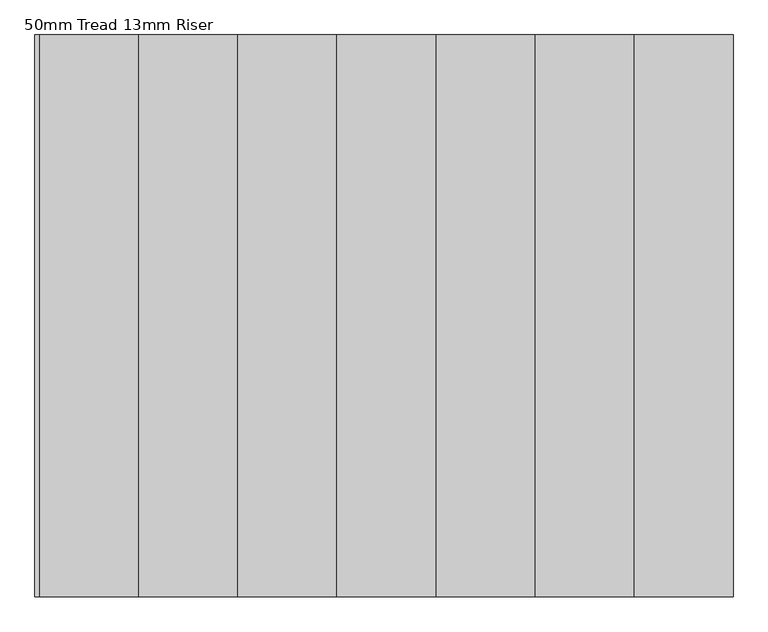
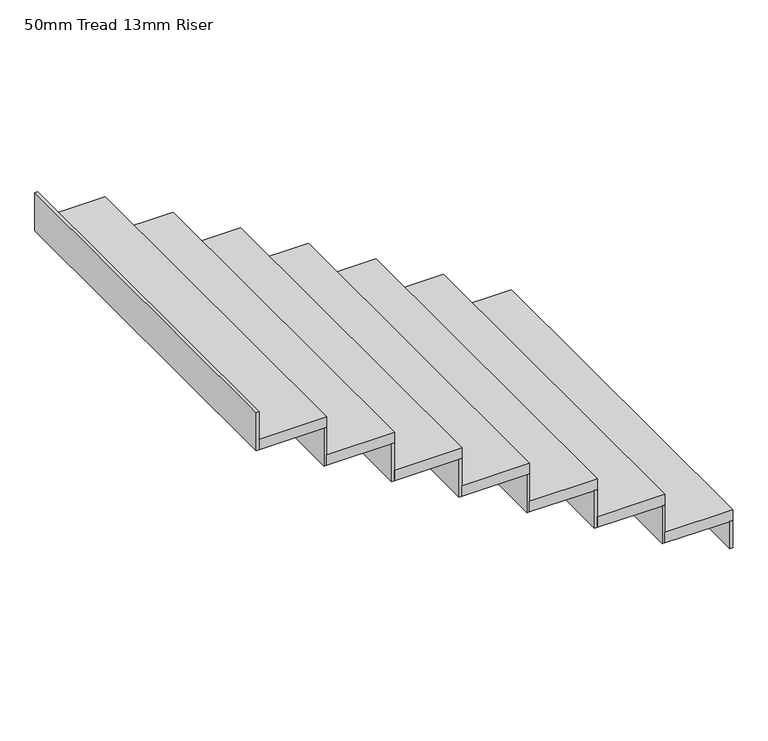
"""IFC4 building model written with IfcOpenShell, lengths in millimetres: stair flight geometry, 50mm Tread 13mm Riser."""

import ifcopenshell
import ifcopenshell.guid

model = None  # the IFC model being written
_history = None  # IfcOwnerHistory: only IFC2X3 demands one
_inside = {}  # id of a spatial element -> (the spatial element, [elements in it])
_under = {}  # id of a project, library or spatial element -> (it, [spatial elements below it])
_declared = {}  # id of a project -> (the project, [libraries it declares])
_typed = {}  # id of a type object -> (the type object, [elements of that type])
_made_of = {}  # id of a material, layer set ... -> (it, [elements and type objects made of it])


def new_model(schema):
    """Start an empty IFC model of exactly this schema.

    Asked for "IFC4X3", IfcOpenShell would pick the latest addendum, in which some entities
    have other attributes; the version numbers below select the first issue.
    IFC2X3 requires an IfcOwnerHistory on every rooted entity: one is made here for all.
    """
    global model, _history
    if schema == "IFC4X3":
        model = ifcopenshell.file(schema_version=(4, 3, 0, 0))
    else:
        model = ifcopenshell.file(schema=schema)
    _inside.clear()
    _under.clear()
    _declared.clear()
    _typed.clear()
    _made_of.clear()
    _history = None
    if model.schema == "IFC2X3":
        org = make("IfcOrganization", Name="unknown")
        user = make(
            "IfcPersonAndOrganization",
            ThePerson=make("IfcPerson", FamilyName="unknown"),
            TheOrganization=org,
        )
        app = make(
            "IfcApplication",
            ApplicationDeveloper=org,
            Version="unknown",
            ApplicationFullName="unknown",
            ApplicationIdentifier="unknown",
        )
        _history = make(
            "IfcOwnerHistory",
            OwningUser=user,
            OwningApplication=app,
            ChangeAction="ADDED",
            CreationDate=0,
        )
    return model


def make(cls, **values):
    """One entity of the class cls with the attributes given. An attribute that is None is left unset."""
    return model.create_entity(
        cls, **{name: value for name, value in values.items() if value is not None}
    )


def rooted(cls, **values):
    """An entity with a GlobalId (a new one), such as an element, a storey or a relation."""
    return make(cls, GlobalId=ifcopenshell.guid.new(), OwnerHistory=_history, **values)


def si_unit(unit_type, name, prefix=None):
    """IfcSIUnit, for example si_unit("LENGTHUNIT", "METRE", prefix="MILLI")."""
    return make("IfcSIUnit", UnitType=unit_type, Prefix=prefix, Name=name)


def assignment(units):
    """IfcUnitAssignment: the units of a project."""
    return None if units is None else make("IfcUnitAssignment", Units=units)


def point(xyz):
    """IfcCartesianPoint."""
    return None if xyz is None else make("IfcCartesianPoint", Coordinates=xyz)


def direction(xyz):
    """IfcDirection."""
    return None if xyz is None else make("IfcDirection", DirectionRatios=xyz)


def frame(location, z_axis=None, x_axis=None):
    """IfcAxis2Placement3D, a coordinate frame: its origin and axes. An axis left out is left unset."""
    return make(
        "IfcAxis2Placement3D",
        Location=point(location),
        Axis=direction(z_axis),
        RefDirection=direction(x_axis),
    )


def origin():
    """The frame at (0, 0, 0) with its axes left unset."""
    return frame((0.0, 0.0, 0.0))


def place(relative_to, where):
    """IfcLocalPlacement: puts the frame where relative to a parent placement (None: the world)."""
    return make(
        "IfcLocalPlacement", PlacementRelTo=relative_to, RelativePlacement=where
    )


def context(
    kind, dimensions, precision=None, world=None, true_north=None, identifier=None
):
    """IfcGeometricRepresentationContext, for example the 3D "Model" context."""
    return make(
        "IfcGeometricRepresentationContext",
        ContextIdentifier=identifier,
        ContextType=kind,
        CoordinateSpaceDimension=dimensions,
        Precision=precision,
        WorldCoordinateSystem=world,
        TrueNorth=true_north,
    )


def project(units=None, contexts=None):
    """IfcProject with its units and contexts."""
    return rooted(
        "IfcProject",
        Name="project",
        RepresentationContexts=contexts,
        UnitsInContext=assignment(units),
    )


def spatial(cls, under=None, at=None, **own):
    """A site, building, storey or space (cls), placed at a placement, below another one or the project."""
    s = rooted(cls, ObjectPlacement=at, **own)
    if under is not None:
        _under.setdefault(under.id(), (under, []))[1].append(s)
    return s


def polyline(points):
    """IfcPolyline through the points."""
    return make("IfcPolyline", Points=[point(p) for p in points])


def outline(outer, holes=None, kind="AREA"):
    """IfcArbitraryClosedProfileDef: a profile drawn as a closed curve; with holes, ...WithVoids."""
    if holes is None:
        return make("IfcArbitraryClosedProfileDef", ProfileType=kind, OuterCurve=outer)
    return make(
        "IfcArbitraryProfileDefWithVoids",
        ProfileType=kind,
        OuterCurve=outer,
        InnerCurves=holes,
    )


def extrude(swept, where, along, depth):
    """IfcExtrudedAreaSolid: the profile swept, set in the frame where, extruded along a direction by depth."""
    return make(
        "IfcExtrudedAreaSolid",
        SweptArea=swept,
        Position=where,
        ExtrudedDirection=direction(along),
        Depth=depth,
    )


def shape(context_of_items, identifier, shape_type, items):
    """IfcShapeRepresentation: the items that make up one representation, for example the "Body"."""
    return make(
        "IfcShapeRepresentation",
        ContextOfItems=context_of_items,
        RepresentationIdentifier=identifier,
        RepresentationType=shape_type,
        Items=items,
    )


def source(mapping_origin, context_of_items, identifier, shape_type, items):
    """IfcRepresentationMap: a shape defined once, which mapped items show again and again."""
    return make(
        "IfcRepresentationMap",
        MappingOrigin=mapping_origin,
        MappedRepresentation=shape(context_of_items, identifier, shape_type, items),
    )


def transform(
    local_origin,
    x_axis=None,
    y_axis=None,
    z_axis=None,
    scale=None,
    scale2=None,
    scale3=None,
    uniform=True,
):
    """IfcCartesianTransformationOperator3D, or its non-uniform kind. x_axis, y_axis, z_axis: its Axis1, 2, 3."""
    if uniform:
        return make(
            "IfcCartesianTransformationOperator3D",
            Axis1=direction(x_axis),
            Axis2=direction(y_axis),
            LocalOrigin=point(local_origin),
            Scale=scale,
            Axis3=direction(z_axis),
        )
    return make(
        "IfcCartesianTransformationOperator3DnonUniform",
        Axis1=direction(x_axis),
        Axis2=direction(y_axis),
        LocalOrigin=point(local_origin),
        Scale=scale,
        Axis3=direction(z_axis),
        Scale2=scale2,
        Scale3=scale3,
    )


def mapped(mapping_source, mapping_target):
    """IfcMappedItem: shows the shape of a source again, moved by a transform."""
    return make(
        "IfcMappedItem", MappingSource=mapping_source, MappingTarget=mapping_target
    )


def made_of(thing, what):
    """Note that an element or type object is made of a material, layer set ...; save() writes the relation."""
    if what is not None:
        _made_of.setdefault(what.id(), (what, []))[1].append(thing)
    return thing


def element(
    cls,
    number,
    at=None,
    inside=None,
    cuts=None,
    type_object=None,
    material=None,
    context=None,
    identifier="Body",
    shape_type=None,
    held_by="IfcProductDefinitionShape",
    body=None,
    shapes=None,
    **own,
):
    """One element of the class cls, such as IfcWall. Its Tag is "e" and its number.

    at: its placement. inside: the storey or other place that contains it. cuts: it is an
    opening in that element (IfcRelVoidsElement). A single representation is given by context,
    identifier, shape_type and body (its items); several are given by shapes. held_by: the class
    of the entity that holds the representations. save() writes the other relations.
    """
    e = rooted(cls, Tag="e%d" % number, ObjectPlacement=at, **own)
    if body is not None:
        shapes = [shape(context, identifier, shape_type, body)]
    if shapes is not None:
        e.Representation = make(held_by, Representations=shapes)
    if inside is not None:
        _inside.setdefault(inside.id(), (inside, []))[1].append(e)
    if cuts is not None:
        rooted(
            "IfcRelVoidsElement", RelatingBuildingElement=cuts, RelatedOpeningElement=e
        )
    if type_object is not None:
        _typed.setdefault(type_object.id(), (type_object, []))[1].append(e)
    return made_of(e, material)


def aggregate(whole, parts):
    """IfcRelAggregates: a whole, such as a stair, and the parts it consists of."""
    return rooted("IfcRelAggregates", RelatingObject=whole, RelatedObjects=parts)


def save(model, path):
    """Write the relations noted so far, then the file.

    IfcRelAggregates (storeys below a building ...), IfcRelContainedInSpatialStructure (elements
    in a storey), IfcRelDefinesByType, IfcRelAssociatesMaterial and IfcRelDeclares: one each for
    every whole, place, type object, material and project.
    """
    for whole, parts in _under.values():
        aggregate(whole, parts)
    for where, things in _inside.values():
        rooted(
            "IfcRelContainedInSpatialStructure",
            RelatedElements=things,
            RelatingStructure=where,
        )
    for kind, things in _typed.values():
        rooted("IfcRelDefinesByType", RelatedObjects=things, RelatingType=kind)
    for what, things in _made_of.values():
        rooted("IfcRelAssociatesMaterial", RelatedObjects=things, RelatingMaterial=what)
    for by, libraries in _declared.values():
        rooted("IfcRelDeclares", RelatingContext=by, RelatedDefinitions=libraries)
    model.write(path)


def stair_flight_50mm_tread_13mm_riser_a4aa0c66(model_context):
    return source(origin(), model_context, "Body", "SweptSolid", [
        extrude(outline(polyline([(-13456.918089, 12730.6768963), (-13444.418089, 12730.6768963), (-13444.418089, 11030.6768963), (-13456.918089, 11030.6768963), (-13456.918089, 12730.6768963)])), frame((0.0, 0.0, -3200.0), z_axis=(0.0, 0.0, 1.0), x_axis=(1.0, 0.0, 0.0)), (0.0, 0.0, 1.0), 127.7777778),
        extrude(outline(polyline([(-13744.418089, 11030.6768963), (-13744.418089, 12730.6768963), (-13444.418089, 12730.6768963), (-13444.418089, 11030.6768963), (-13744.418089, 11030.6768963)])), frame((0.0, 0.0, -3072.2222222), z_axis=(0.0, 0.0, 1.0), x_axis=(1.0, 0.0, 0.0)), (0.0, 0.0, 1.0), 50.0),
        extrude(outline(polyline([(-13756.918089, 12730.6768963), (-13744.418089, 12730.6768963), (-13744.418089, 11030.6768963), (-13756.918089, 11030.6768963), (-13756.918089, 12730.6768963)])), frame((0.0, 0.0, -3072.2222222), z_axis=(0.0, 0.0, 1.0), x_axis=(1.0, 0.0, 0.0)), (0.0, 0.0, 1.0), 177.7777778),
        extrude(outline(polyline([(-14044.418089, 11030.6768963), (-14044.418089, 12730.6768963), (-13744.418089, 12730.6768963), (-13744.418089, 11030.6768963), (-14044.418089, 11030.6768963)])), frame((0.0, 0.0, -2894.4444444), z_axis=(0.0, 0.0, 1.0), x_axis=(1.0, 0.0, 0.0)), (0.0, 0.0, 1.0), 50.0),
        extrude(outline(polyline([(-14056.918089, 12730.6768963), (-14044.418089, 12730.6768963), (-14044.418089, 11030.6768963), (-14056.918089, 11030.6768963), (-14056.918089, 12730.6768963)])), frame((0.0, 0.0, -2894.4444444), z_axis=(0.0, 0.0, 1.0), x_axis=(1.0, 0.0, 0.0)), (0.0, 0.0, 1.0), 177.7777778),
        extrude(outline(polyline([(-14344.418089, 11030.6768963), (-14344.418089, 12730.6768963), (-14044.418089, 12730.6768963), (-14044.418089, 11030.6768963), (-14344.418089, 11030.6768963)])), frame((0.0, 0.0, -2716.6666667), z_axis=(0.0, 0.0, 1.0), x_axis=(1.0, 0.0, 0.0)), (0.0, 0.0, 1.0), 50.0),
        extrude(outline(polyline([(-14356.918089, 12730.6768963), (-14344.418089, 12730.6768963), (-14344.418089, 11030.6768963), (-14356.918089, 11030.6768963), (-14356.918089, 12730.6768963)])), frame((0.0, 0.0, -2716.6666667), z_axis=(0.0, 0.0, 1.0), x_axis=(1.0, 0.0, 0.0)), (0.0, 0.0, 1.0), 177.7777778),
        extrude(outline(polyline([(-14644.418089, 11030.6768963), (-14644.418089, 12730.6768963), (-14344.418089, 12730.6768963), (-14344.418089, 11030.6768963), (-14644.418089, 11030.6768963)])), frame((0.0, 0.0, -2538.8888889), z_axis=(0.0, 0.0, 1.0), x_axis=(1.0, 0.0, 0.0)), (0.0, 0.0, 1.0), 50.0),
        extrude(outline(polyline([(-14656.918089, 12730.6768963), (-14644.418089, 12730.6768963), (-14644.418089, 11030.6768963), (-14656.918089, 11030.6768963), (-14656.918089, 12730.6768963)])), frame((0.0, 0.0, -2538.8888889), z_axis=(0.0, 0.0, 1.0), x_axis=(1.0, 0.0, 0.0)), (0.0, 0.0, 1.0), 177.7777778),
        extrude(outline(polyline([(-14944.418089, 11030.6768963), (-14944.418089, 12730.6768963), (-14644.418089, 12730.6768963), (-14644.418089, 11030.6768963), (-14944.418089, 11030.6768963)])), frame((0.0, 0.0, -2361.1111111), z_axis=(0.0, 0.0, 1.0), x_axis=(1.0, 0.0, 0.0)), (0.0, 0.0, 1.0), 50.0),
        extrude(outline(polyline([(-14956.918089, 12730.6768963), (-14944.418089, 12730.6768963), (-14944.418089, 11030.6768963), (-14956.918089, 11030.6768963), (-14956.918089, 12730.6768963)])), frame((0.0, 0.0, -2361.1111111), z_axis=(0.0, 0.0, 1.0), x_axis=(1.0, 0.0, 0.0)), (0.0, 0.0, 1.0), 177.7777778),
        extrude(outline(polyline([(-15244.418089, 11030.6768963), (-15244.418089, 12730.6768963), (-14944.418089, 12730.6768963), (-14944.418089, 11030.6768963), (-15244.418089, 11030.6768963)])), frame((0.0, 0.0, -2183.3333333), z_axis=(0.0, 0.0, 1.0), x_axis=(1.0, 0.0, 0.0)), (0.0, 0.0, 1.0), 50.0),
        extrude(outline(polyline([(-15256.918089, 12730.6768963), (-15244.418089, 12730.6768963), (-15244.418089, 11030.6768963), (-15256.918089, 11030.6768963), (-15256.918089, 12730.6768963)])), frame((0.0, 0.0, -2183.3333333), z_axis=(0.0, 0.0, 1.0), x_axis=(1.0, 0.0, 0.0)), (0.0, 0.0, 1.0), 177.7777778),
        extrude(outline(polyline([(-15556.918089, 12730.6768963), (-15544.418089, 12730.6768963), (-15544.418089, 11030.6768963), (-15556.918089, 11030.6768963), (-15556.918089, 12730.6768963)])), frame((0.0, 0.0, -2005.5555556), z_axis=(0.0, 0.0, 1.0), x_axis=(1.0, 0.0, 0.0)), (0.0, 0.0, 1.0), 177.7777778),
        extrude(outline(polyline([(-15544.418089, 11030.6768963), (-15544.418089, 12730.6768963), (-15244.418089, 12730.6768963), (-15244.418089, 11030.6768963), (-15544.418089, 11030.6768963)])), frame((0.0, 0.0, -2005.5555556), z_axis=(0.0, 0.0, 1.0), x_axis=(1.0, 0.0, 0.0)), (0.0, 0.0, 1.0), 50.0),
    ])


if __name__ == "__main__":
    model = new_model("IFC4")
    model_context = context("Model", 3, world=origin())
    ifc_project = project(units=[si_unit("LENGTHUNIT", "METRE", prefix="MILLI")], contexts=[model_context])
    site = spatial("IfcSite", under=ifc_project)
    building = spatial("IfcBuilding", under=site)
    placement = place(None, origin())
    stair_flight_50mm_tread_13mm_riser_shape = stair_flight_50mm_tread_13mm_riser_a4aa0c66(model_context)
    element("IfcStairFlight", 1, ObjectType="50mm Tread 13mm Riser", at=placement, inside=building, context=model_context, shape_type="MappedRepresentation", body=[
        mapped(stair_flight_50mm_tread_13mm_riser_shape, transform((0.0, 0.0, 0.0), x_axis=(1.0, 0.0, 0.0), y_axis=(0.0, 1.0, 0.0), z_axis=(0.0, 0.0, 1.0))),
    ])
    save(model, "model.ifc")
